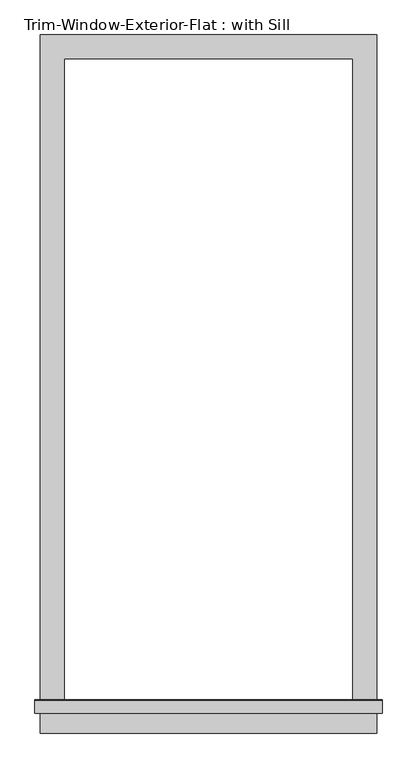
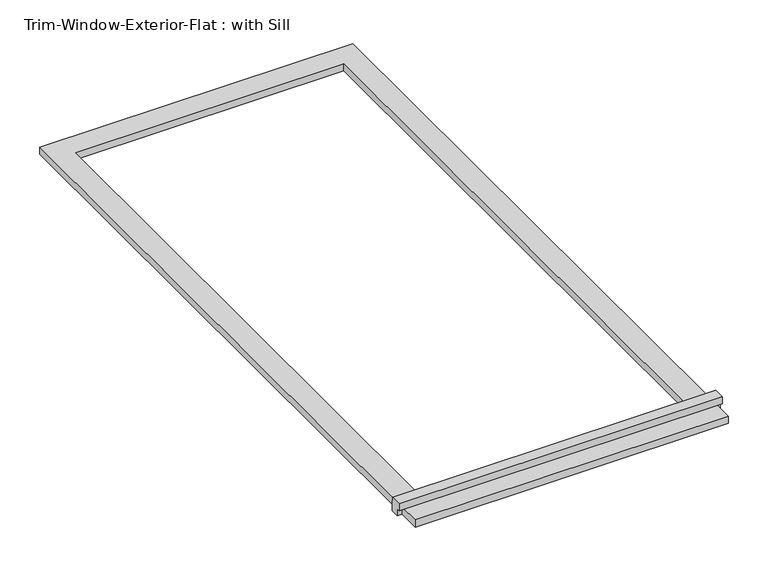
"""IFC4 building model written with IfcOpenShell, lengths in millimetres: proxy geometry, Trim-Window-Exterior-Flat : with Sill."""

from ifc_helpers import new_model, si_unit, frame, origin, origin_with_axes, place, context, project, spatial, polyline, outline, extrude, source, transform, mapped, element, save


def trim_window_exterior_flat_with_sill_2ae81710(model_context):
    return source(origin(), model_context, "Body", "SweptSolid", [
        extrude(outline(polyline([(400.05, -1546.1823709), (400.05, -1603.3323709), (-400.05, -1603.3323709), (-400.05, -1546.1823709), (400.05, -1546.1823709)])), origin_with_axes(), (0.0, 0.0, 1.0), 19.05),
        extrude(outline(polyline([(-1555.75, 38.1), (-1526.4580645, 38.1), (-1524.0, 19.05), (-1524.0, 0.0), (-1546.1823709, 0.0), (-1546.1823709, 19.05), (-1555.75, 19.05), (-1555.75, 38.1)])), frame((-412.75, 0.0, 0.0), z_axis=(1.0, 0.0, 0.0), x_axis=(0.0, 1.0, 0.0)), (0.0, 0.0, 1.0), 825.5),
        extrude(outline(polyline([(-400.05, 57.15), (400.05, 57.15), (400.05, -1524.0), (342.9, -1524.0), (342.9, 0.0), (-342.9, 0.0), (-342.9, -1524.0), (-400.05, -1524.0), (-400.05, 57.15)])), origin_with_axes(), (0.0, 0.0, 1.0), 19.05),
    ])


if __name__ == "__main__":
    model = new_model("IFC4")
    model_context = context("Model", 3, world=origin())
    ifc_project = project(units=[si_unit("LENGTHUNIT", "METRE", prefix="MILLI")], contexts=[model_context])
    site = spatial("IfcSite", under=ifc_project)
    building = spatial("IfcBuilding", under=site)
    placement = place(None, origin())
    trim_window_exterior_flat_with_sill_shape = trim_window_exterior_flat_with_sill_2ae81710(model_context)
    element("IfcBuildingElementProxy", 1, Name="Trim-Window-Exterior-Flat : with Sill", ObjectType="Trim-Window-Exterior-Flat : with Sill", at=placement, inside=building, context=model_context, shape_type="MappedRepresentation", body=[
        mapped(trim_window_exterior_flat_with_sill_shape, transform((0.0, 0.0, 0.0), x_axis=(1.0, 0.0, 0.0), y_axis=(0.0, 1.0, 0.0), z_axis=(0.0, 0.0, 1.0))),
    ])
    save(model, "model.ifc")

# Revit data of these elements
# Type "Trim-Window-Exterior-Flat : with Sill"
#   Trim Width = 0' - 2 1/4"
#   Trim Thickness_Picture Frame = 0' - 1 1/4"
#   Trim Thickness_with Sill = 0' - 0 3/4"
#   Sill Thickness = 0' - 1 1/4"
#   Opening Width [instance default] = 2' - 0"
#   Opening Height [instance default] = 3' - 0"
#   Default Elevation = 4' - 0"
#   Sill = yes
#   Picture Frame = no
#   Trim Material [instance default] = none
# Element 1 (IfcBuildingElementProxy, "Trim-Window-Exterior-Flat : with Sill")
#   Opening Width = 2' - 3"
#   Opening Height = 5' - 0"
#   Trim Material = Clad - White
#   Materials on its faces: "Clad - White"
# Materials
#   "Clad - White": class "Wood", colour RGB 242 242 238, transparency 0, Cost = 0
